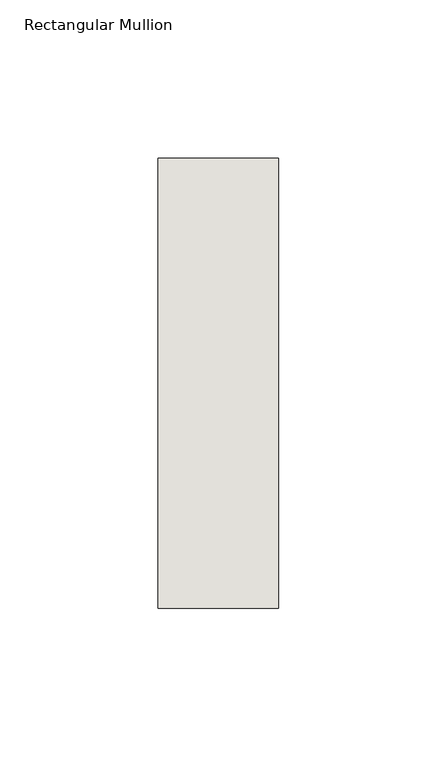
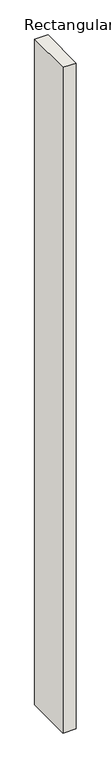
"""IFC4 building model written with IfcOpenShell, lengths in millimetres: wall geometry, Rectangular Mullion : NLRS_21_CWM_hsb-regel 38x142_gen_rsf."""

from ifc_helpers import new_model, si_unit, frame, origin, place, context, project, spatial, polyline, outline, extrude, source, transform, mapped, element, save


def rectangular_mullion_df2c1bf7(model_context):
    return source(origin(), model_context, "Body", "SweptSolid", [
        extrude(outline(polyline([(0.0, -71.0), (-38.0, -71.0), (-38.0, 71.0), (0.0, 71.0), (0.0, -71.0)])), frame((0.0, 0.0, -2038.0), z_axis=(0.0, 0.0, 1.0), x_axis=(1.0, 0.0, 0.0)), (0.0, 0.0, 1.0), 2038.0),
    ])


if __name__ == "__main__":
    model = new_model("IFC4")
    model_context = context("Model", 3, world=origin())
    ifc_project = project(units=[si_unit("LENGTHUNIT", "METRE", prefix="MILLI")], contexts=[model_context])
    site = spatial("IfcSite", under=ifc_project)
    building = spatial("IfcBuilding", under=site)
    placement = place(None, origin())
    rectangular_mullion_shape = rectangular_mullion_df2c1bf7(model_context)
    element("IfcWall", 1, ObjectType="Rectangular Mullion : NLRS_21_CWM_hsb-regel 38x142_gen_rsf", at=placement, inside=building, context=model_context, shape_type="MappedRepresentation", body=[
        mapped(rectangular_mullion_shape, transform((0.0, 0.0, 0.0), x_axis=(1.0, 0.0, 0.0), y_axis=(0.0, 1.0, 0.0), z_axis=(0.0, 0.0, 1.0))),
    ])
    save(model, "model.ifc")

# Revit data of these elements
# Type "Rectangular Mullion : NLRS_21_CWM_hsb-regel 38x142_gen_rsf"
#   Type IfcGUID = "07M7mRoiH1CR8m_RSKIwpF"
#   Assembly Code = "21.10"
#   IfcExportAs = "IfcWall"
#   built-in parameter 1007322 = 0.465879 (stored number, unit not read)
#   built-in parameter 1007321 = 0.062336 (stored number, unit not read)
#   built-in parameter 1007320 = 0.062336 (stored number, unit not read)
# Element 1 (IfcWall, "Rectangular Mullion : NLRS_21_CWM_hsb-regel 38x142_gen_rsf")
#   Materials on its faces: "NLRS_i2_hout naaldhout vuren_gen_rsf"
# Materials
#   "NLRS_i2_hout naaldhout vuren_gen_rsf": class "I - Hout", colour RGB 234 199 147, transparency 0, Keynote = "i2", Manufacturer = "Revit Standards Foundation", URL = "www.revitstandards.org", Description = "hout vuren", Cost = 0
